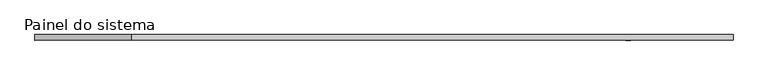
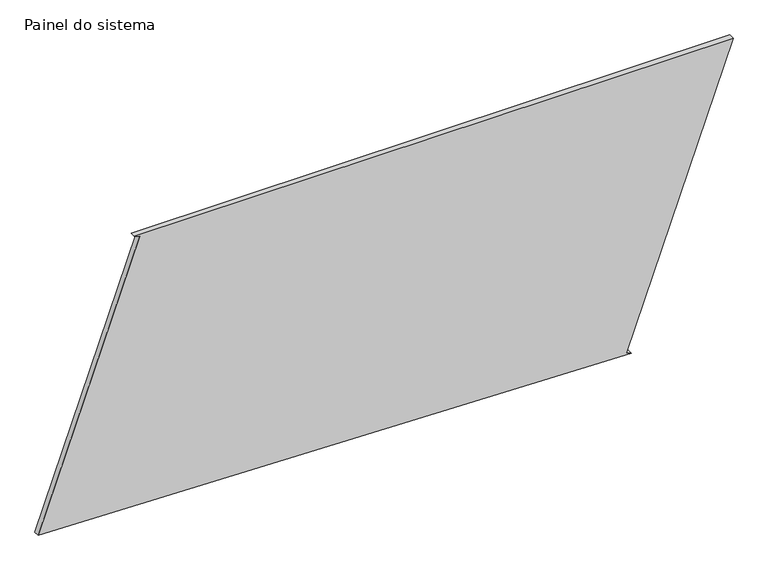
"""IFC4 building model written with IfcOpenShell, lengths in millimetres: plate geometry, Painel do sistema : Envidraçado."""

from ifc_helpers import new_model, si_unit, frame, origin, place, context, project, spatial, polyline, outline, extrude, source, transform, mapped, element, save


def painel_do_sistema_eb4efb99(model_context):
    return source(origin(), model_context, "Body", "SweptSolid", [
        extrude(outline(polyline([(0.0, 1111.8075043), (8.505028, 1088.2986869), (1346.547191, 1572.376037), (1346.547191, -1136.8509815), (1338.042163, -1113.342164), (69.22288, -1572.376037), (0.0, 1111.8075043)])), frame((0.0, 24.5, 0.0), z_axis=(0.0, 1.0, 0.0), x_axis=(0.0, 0.0, 1.0)), (0.0, 0.0, 1.0), 25.0),
    ])


if __name__ == "__main__":
    model = new_model("IFC4")
    model_context = context("Model", 3, world=origin())
    ifc_project = project(units=[si_unit("LENGTHUNIT", "METRE", prefix="MILLI")], contexts=[model_context])
    site = spatial("IfcSite", under=ifc_project)
    building = spatial("IfcBuilding", under=site)
    placement = place(None, origin())
    painel_do_sistema_shape = painel_do_sistema_eb4efb99(model_context)
    element("IfcPlate", 1, ObjectType="Painel do sistema : Envidraçado", at=placement, inside=building, context=model_context, shape_type="MappedRepresentation", body=[
        mapped(painel_do_sistema_shape, transform((0.0, 0.0, 0.0), x_axis=(1.0, 0.0, 0.0), y_axis=(0.0, 1.0, 0.0), z_axis=(0.0, 0.0, 1.0))),
    ])
    save(model, "model.ifc")

# Revit data of these elements
# Type "Painel do sistema : Envidraçado"
#   Construction Type Id = "GSP4R"
#   Analytic Construction = "Vidraça única Pilkington 1/8 pol"
#   Visual Light Transmittance = 0.9
#   Solar Heat Gain Coefficient = 0.86
#   Heat Transfer Coefficient (U) = 6.7069 W/(m²·K)
# Element 1 (IfcPlate, "Painel do sistema : Envidraçado")
#   Materials on its faces: "Vidro"
# Materials
#   "Vidro": class "Vidro", colour RGB 0 128 192, transparency 0.9, Description = "Vidro de sílica", Cost = 0
